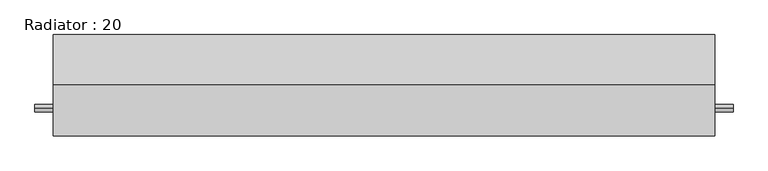
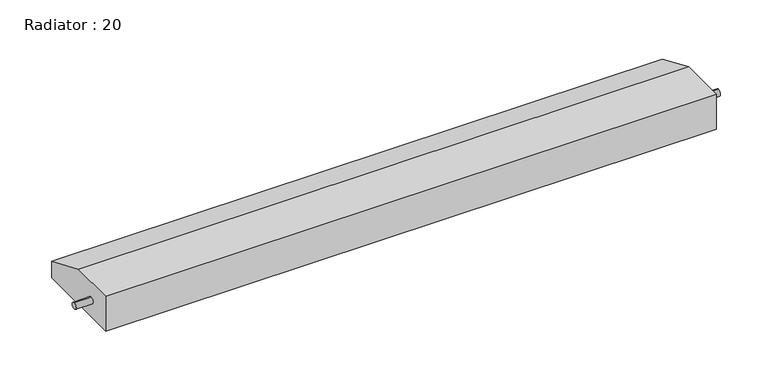
"""IFC4 building model written with IfcOpenShell, lengths in millimetres: proxy geometry, Radiator : 20."""

from ifc_helpers import new_model, si_unit, frame, origin, place, context, project, spatial, circle_curve, source, transform, mapped, element, save
from ifc_brep_helpers import plane_surface, cylinder_surface, advanced_brep


def radiator_20_f1613ed5(model_context):
    return source(origin(), model_context, "Body", "AdvancedBrep", [
        advanced_brep(
        [(915.0, 280.0, 0.0), (915.0, 280.0, 52.3875), (915.0, 141.8875, 111.125), (915.0, 0.0, 111.125), (915.0, 0.0, 0.0), (915.0, 76.2, 42.3875), (915.0, 76.2, 62.3875), (-915.0, 280.0, 0.0), (-915.0, 0.0, 0.0), (-915.0, 0.0, 111.125), (-915.0, 141.8875, 111.125), (-915.0, 280.0, 52.3875), (-915.0, 76.2, 62.3875), (-915.0, 76.2, 42.3875), (-965.8, 76.2, 42.3875), (-965.8, 76.2, 62.3875), (965.8, 76.2, 42.3875), (965.8, 76.2, 62.3875)],
        [
            (0, 1),
            (1, 2),
            (2, 3),
            (3, 4),
            (4, 0),
            (5, 6, circle_curve(frame((915.0, 76.2, 52.3875), z_axis=(-1.0, 0.0, 0.0), x_axis=(0.0, 0.0, 1.0)), 10.0)),
            (6, 5, circle_curve(frame((915.0, 76.2, 52.3875), z_axis=(-1.0, 0.0, 0.0), x_axis=(0.0, 0.0, 1.0)), 10.0)),
            (7, 8),
            (8, 9),
            (9, 10),
            (10, 11),
            (11, 7),
            (12, 13, circle_curve(frame((-915.0, 76.2, 52.3875), z_axis=(1.0, 0.0, 0.0), x_axis=(0.0, 0.0, 1.0)), 10.0)),
            (13, 12, circle_curve(frame((-915.0, 76.2, 52.3875), z_axis=(1.0, 0.0, 0.0), x_axis=(0.0, 0.0, 1.0)), 10.0)),
            (0, 7),
            (11, 1),
            (10, 2),
            (9, 3),
            (8, 4),
            (14, 15, circle_curve(frame((-965.8, 76.2, 52.3875), z_axis=(-1.0, 0.0, 0.0), x_axis=(0.0, 0.0, 1.0)), 10.0)),
            (15, 14, circle_curve(frame((-965.8, 76.2, 52.3875), z_axis=(-1.0, 0.0, 0.0), x_axis=(0.0, 0.0, 1.0)), 10.0)),
            (16, 17, circle_curve(frame((965.8, 76.2, 52.3875), z_axis=(1.0, 0.0, 0.0), x_axis=(0.0, 0.0, 1.0)), 10.0)),
            (17, 16, circle_curve(frame((965.8, 76.2, 52.3875), z_axis=(1.0, 0.0, 0.0), x_axis=(0.0, 0.0, 1.0)), 10.0)),
            (14, 13),
            (12, 15),
            (17, 6),
            (5, 16),
        ],
        [
            plane_surface(frame((915.0, 280.0, 0.0), z_axis=(1.0, 0.0, 0.0), x_axis=(0.0, 0.0, 1.0))),
            plane_surface(frame((-915.0, 280.0, 0.0), z_axis=(-1.0, 0.0, 0.0), x_axis=(0.0, 0.0, -1.0))),
            plane_surface(frame((915.0, 280.0, 0.0), z_axis=(0.0, 1.0, 0.0), x_axis=(-1.0, 0.0, 0.0))),
            plane_surface(frame((915.0, 280.0, 52.3875), z_axis=(0.0, 0.3913646080488335, 0.9202357000066793), x_axis=(-1.0, 0.0, 0.0))),
            plane_surface(frame((915.0, 141.8875, 111.125), z_axis=(0.0, 0.0, 1.0), x_axis=(-1.0, 0.0, 0.0))),
            plane_surface(frame((915.0, 0.0, 111.125), z_axis=(0.0, -1.0, 0.0), x_axis=(-1.0, 0.0, 0.0))),
            plane_surface(frame((915.0, 0.0, 0.0), z_axis=(0.0, 0.0, -1.0), x_axis=(-1.0, 0.0, 0.0))),
            plane_surface(frame((-965.8, 76.2, 62.3875), z_axis=(-1.0, 0.0, 0.0), x_axis=(0.0, 1.0, 0.0))),
            plane_surface(frame((965.8, 76.2, 62.3875), z_axis=(1.0, 0.0, 0.0), x_axis=(0.0, -1.0, 0.0))),
            cylinder_surface(frame((965.8, 76.2, 52.3875), z_axis=(-1.0, 0.0, 0.0), x_axis=(0.0, 0.0, 1.0)), 10.0),
        ],
        [
            (0, [[1, 2, 3, 4, 5], [6, 7]]),
            (1, [[8, 9, 10, 11, 12], [13, 14]]),
            (2, [[-1, 15, -12, 16]]),
            (3, [[-2, -16, -11, 17]]),
            (4, [[-3, -17, -10, 18]]),
            (5, [[-4, -18, -9, 19]]),
            (6, [[-5, -19, -8, -15]]),
            (7, [[20, 21]]),
            (8, [[22, 23]]),
            (9, [[-20, 24, -13, 25]]),
            (9, [[-23, 26, -6, 27]]),
            (9, [[-21, -25, -14, -24]]),
            (9, [[-22, -27, -7, -26]]),
        ],
    ),
    ])


if __name__ == "__main__":
    model = new_model("IFC4")
    model_context = context("Model", 3, world=origin())
    ifc_project = project(units=[si_unit("LENGTHUNIT", "METRE", prefix="MILLI")], contexts=[model_context])
    site = spatial("IfcSite", under=ifc_project)
    building = spatial("IfcBuilding", under=site)
    placement = place(None, origin())
    radiator_20_shape = radiator_20_f1613ed5(model_context)
    element("IfcBuildingElementProxy", 1, Name="Radiator : 20", ObjectType="Radiator : 20", at=placement, inside=building, context=model_context, shape_type="MappedRepresentation", body=[
        mapped(radiator_20_shape, transform((0.0, 0.0, 0.0), x_axis=(1.0, 0.0, 0.0), y_axis=(0.0, 1.0, 0.0), z_axis=(0.0, 0.0, 1.0))),
    ])
    save(model, "model.ifc")

# Revit data of these elements
# Project information
#   Project Issue Date = "Issue Date"
#   Project Status = "Project Status"
#   Client Name = "Owner"
#   Project Address = "Enter address here"
#   Project Name = "Lake Geneva"
#   Project Number = "Project Number"
# Type "Radiator : 20"
#   Type Mark = "RD-01"
#   Pressure Drop [instance default] = 0.000133435 psi
#   Power [instance default] = 4916.71 Btu/h
#   Length [instance default] = 1830 mm
#   Height = 280 mm
#   Flow [instance default] = 228.403 GPM
#   Default Elevation = 100 mm
#   Connector = 0.3937"
#   BtuPerFt = 818.914 Btu/h
#   Assembly Code = ""
